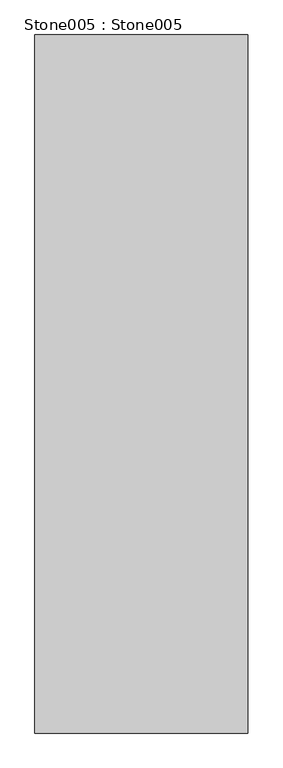
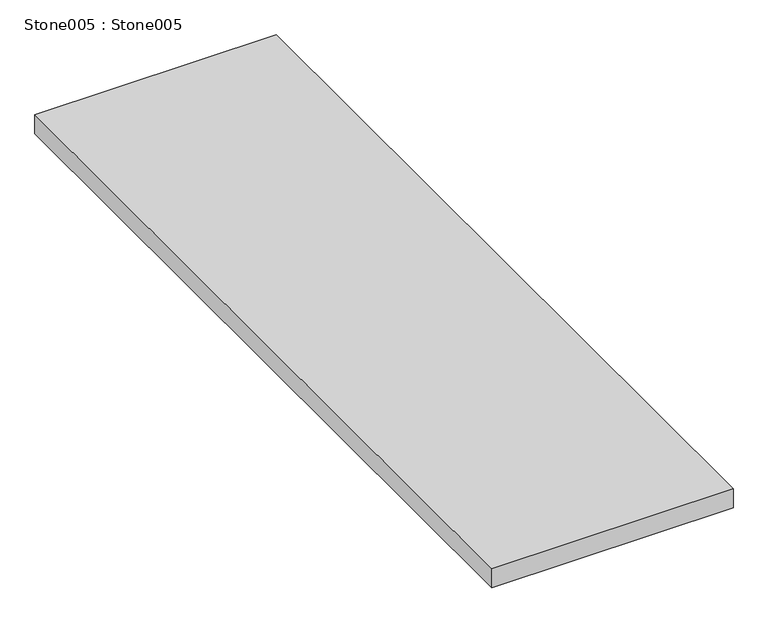
"""IFC4 building model written with IfcOpenShell, lengths in millimetres: proxy geometry, Stone005 : Stone005."""

from ifc_helpers import new_model, si_unit, frame, origin, place, context, project, spatial, polyline, outline, extrude, source, transform, mapped, element, save


def stone005_stone005_4e1e5a6c(model_context):
    return source(origin(), model_context, "Body", "SweptSolid", [
        extrude(outline(polyline([(-2368.8555782, -1052.8906574), (-2978.4555782, -1052.8906574), (-2978.4555782, 947.1093426), (-2368.8555782, 947.1093426), (-2368.8555782, -1052.8906574)])), frame((0.0, 0.0, 36518.596), z_axis=(0.0, 0.0, 1.0), x_axis=(1.0, 0.0, 0.0)), (0.0, 0.0, 1.0), 50.8),
    ])


if __name__ == "__main__":
    model = new_model("IFC4")
    model_context = context("Model", 3, world=origin())
    ifc_project = project(units=[si_unit("LENGTHUNIT", "METRE", prefix="MILLI")], contexts=[model_context])
    site = spatial("IfcSite", under=ifc_project)
    building = spatial("IfcBuilding", under=site)
    placement = place(None, origin())
    stone005_stone005_shape = stone005_stone005_4e1e5a6c(model_context)
    element("IfcBuildingElementProxy", 1, Name="Stone005 : Stone005", ObjectType="Stone005 : Stone005", at=placement, inside=building, context=model_context, shape_type="MappedRepresentation", body=[
        mapped(stone005_stone005_shape, transform((0.0, 0.0, 0.0), x_axis=(1.0, 0.0, 0.0), y_axis=(0.0, 1.0, 0.0), z_axis=(0.0, 0.0, 1.0))),
    ])
    save(model, "model.ifc")

# Revit data of these elements
# Type "Stone005 : Stone005"
#   NameOverride = "Stone005"
# Element 1 (IfcBuildingElementProxy, "Stone005 : Stone005")
#   Materials on its faces: "2\" STONE DECK TBD"
# Materials
#   "2\" STONE DECK TBD": class "Unassigned", colour RGB 199 185 173, transparency 0
